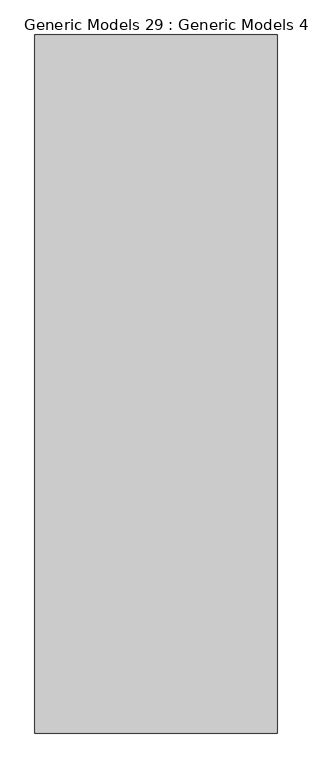
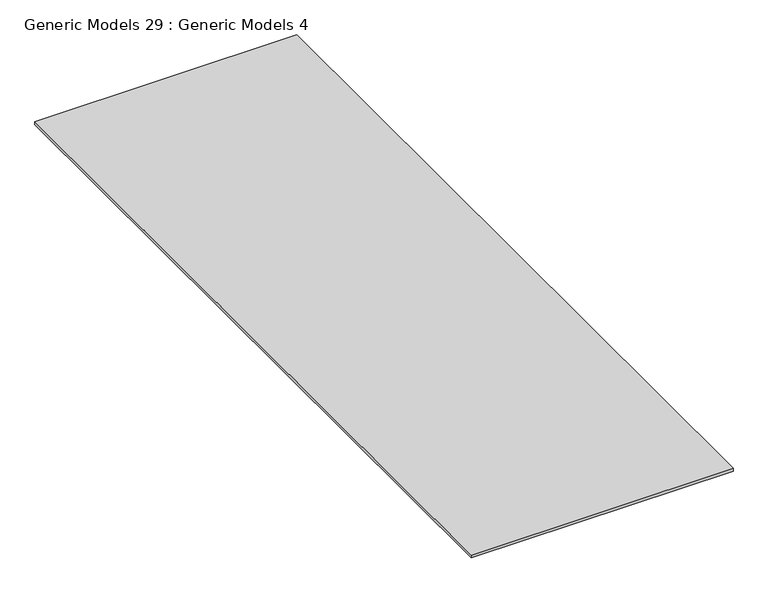
"""IFC4 building model written with IfcOpenShell, lengths in millimetres: proxy geometry, Generic Models 29 : Generic Models 4."""

from ifc_helpers import new_model, si_unit, frame, origin, place, context, project, spatial, polyline, outline, extrude, source, transform, mapped, element, save


def generic_models_29_generic_models_4_b95f0caa(model_context):
    return source(origin(), model_context, "Body", "SweptSolid", [
        extrude(outline(polyline([(8575.5013705, 7054.2769662), (6937.2013704, 7054.2769662), (6937.2013704, 11778.6769662), (8575.5013705, 11778.6769662), (8575.5013705, 7054.2769662)])), frame((0.0, 0.0, 126771.146), z_axis=(0.0, 0.0, 1.0), x_axis=(1.0, 0.0, 0.0)), (0.0, 0.0, 1.0), 19.05),
    ])


if __name__ == "__main__":
    model = new_model("IFC4")
    model_context = context("Model", 3, world=origin())
    ifc_project = project(units=[si_unit("LENGTHUNIT", "METRE", prefix="MILLI")], contexts=[model_context])
    site = spatial("IfcSite", under=ifc_project)
    building = spatial("IfcBuilding", under=site)
    placement = place(None, origin())
    generic_models_29_generic_models_4_shape = generic_models_29_generic_models_4_b95f0caa(model_context)
    element("IfcBuildingElementProxy", 1, Name="Generic Models 29 : Generic Models 4", ObjectType="Generic Models 29 : Generic Models 4", at=placement, inside=building, context=model_context, shape_type="MappedRepresentation", body=[
        mapped(generic_models_29_generic_models_4_shape, transform((0.0, 0.0, 0.0), x_axis=(1.0, 0.0, 0.0), y_axis=(0.0, 1.0, 0.0), z_axis=(0.0, 0.0, 1.0))),
    ])
    save(model, "model.ifc")

# Revit data of these elements
# Element 1 (IfcBuildingElementProxy, "Generic Models 29 : Generic Models 4")
#   Materials on its faces: "_CDX PLYWOOD - SEE STRUCT DWGs"
# Materials
#   "_CDX PLYWOOD - SEE STRUCT DWGs": class "Generic", colour RGB 98 75 74, transparency 0, Cost = 0
